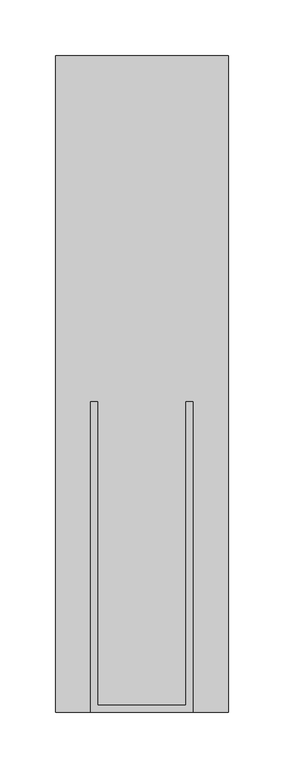
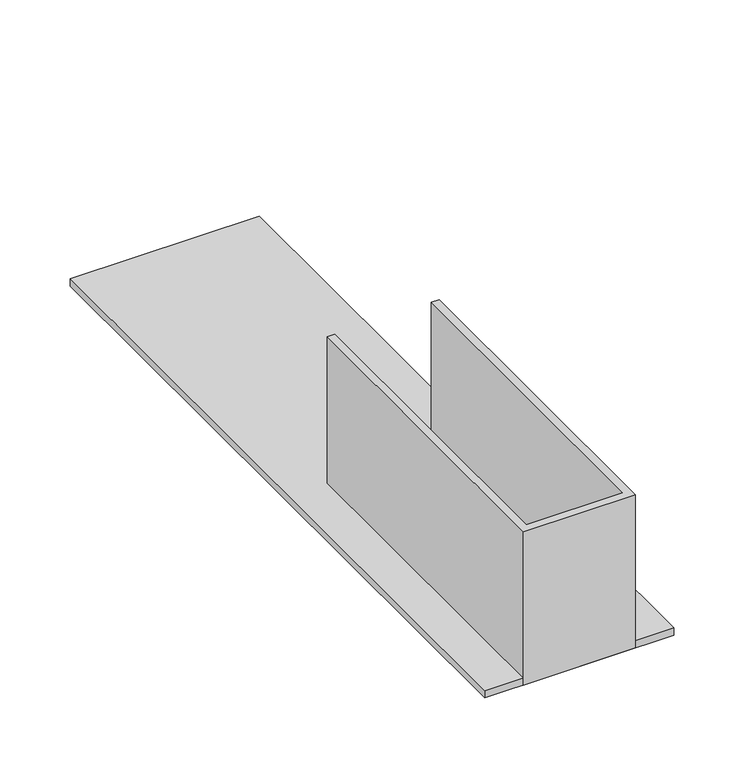
"""IFC4 building model written with IfcOpenShell, lengths in millimetres: fastener geometry, SIMPSON -THGBV - Truss Girder Hanger : SIMPSON -THGBV3.62/11 - HDG."""

import ifcopenshell
import ifcopenshell.guid

model = None  # the IFC model being written
_history = None  # IfcOwnerHistory: only IFC2X3 demands one
_inside = {}  # id of a spatial element -> (the spatial element, [elements in it])
_under = {}  # id of a project, library or spatial element -> (it, [spatial elements below it])
_declared = {}  # id of a project -> (the project, [libraries it declares])
_typed = {}  # id of a type object -> (the type object, [elements of that type])
_made_of = {}  # id of a material, layer set ... -> (it, [elements and type objects made of it])


def new_model(schema):
    """Start an empty IFC model of exactly this schema.

    Asked for "IFC4X3", IfcOpenShell would pick the latest addendum, in which some entities
    have other attributes; the version numbers below select the first issue.
    IFC2X3 requires an IfcOwnerHistory on every rooted entity: one is made here for all.
    """
    global model, _history
    if schema == "IFC4X3":
        model = ifcopenshell.file(schema_version=(4, 3, 0, 0))
    else:
        model = ifcopenshell.file(schema=schema)
    _inside.clear()
    _under.clear()
    _declared.clear()
    _typed.clear()
    _made_of.clear()
    _history = None
    if model.schema == "IFC2X3":
        org = make("IfcOrganization", Name="unknown")
        user = make(
            "IfcPersonAndOrganization",
            ThePerson=make("IfcPerson", FamilyName="unknown"),
            TheOrganization=org,
        )
        app = make(
            "IfcApplication",
            ApplicationDeveloper=org,
            Version="unknown",
            ApplicationFullName="unknown",
            ApplicationIdentifier="unknown",
        )
        _history = make(
            "IfcOwnerHistory",
            OwningUser=user,
            OwningApplication=app,
            ChangeAction="ADDED",
            CreationDate=0,
        )
    return model


def make(cls, **values):
    """One entity of the class cls with the attributes given. An attribute that is None is left unset."""
    return model.create_entity(
        cls, **{name: value for name, value in values.items() if value is not None}
    )


def rooted(cls, **values):
    """An entity with a GlobalId (a new one), such as an element, a storey or a relation."""
    return make(cls, GlobalId=ifcopenshell.guid.new(), OwnerHistory=_history, **values)


def si_unit(unit_type, name, prefix=None):
    """IfcSIUnit, for example si_unit("LENGTHUNIT", "METRE", prefix="MILLI")."""
    return make("IfcSIUnit", UnitType=unit_type, Prefix=prefix, Name=name)


def assignment(units):
    """IfcUnitAssignment: the units of a project."""
    return None if units is None else make("IfcUnitAssignment", Units=units)


def point(xyz):
    """IfcCartesianPoint."""
    return None if xyz is None else make("IfcCartesianPoint", Coordinates=xyz)


def direction(xyz):
    """IfcDirection."""
    return None if xyz is None else make("IfcDirection", DirectionRatios=xyz)


def frame(location, z_axis=None, x_axis=None):
    """IfcAxis2Placement3D, a coordinate frame: its origin and axes. An axis left out is left unset."""
    return make(
        "IfcAxis2Placement3D",
        Location=point(location),
        Axis=direction(z_axis),
        RefDirection=direction(x_axis),
    )


def origin():
    """The frame at (0, 0, 0) with its axes left unset."""
    return frame((0.0, 0.0, 0.0))


def origin_with_axes():
    """The frame at (0, 0, 0) with the z axis (0, 0, 1) and the x axis (1, 0, 0) written out."""
    return frame((0.0, 0.0, 0.0), z_axis=(0.0, 0.0, 1.0), x_axis=(1.0, 0.0, 0.0))


def place(relative_to, where):
    """IfcLocalPlacement: puts the frame where relative to a parent placement (None: the world)."""
    return make(
        "IfcLocalPlacement", PlacementRelTo=relative_to, RelativePlacement=where
    )


def context(
    kind, dimensions, precision=None, world=None, true_north=None, identifier=None
):
    """IfcGeometricRepresentationContext, for example the 3D "Model" context."""
    return make(
        "IfcGeometricRepresentationContext",
        ContextIdentifier=identifier,
        ContextType=kind,
        CoordinateSpaceDimension=dimensions,
        Precision=precision,
        WorldCoordinateSystem=world,
        TrueNorth=true_north,
    )


def project(units=None, contexts=None):
    """IfcProject with its units and contexts."""
    return rooted(
        "IfcProject",
        Name="project",
        RepresentationContexts=contexts,
        UnitsInContext=assignment(units),
    )


def spatial(cls, under=None, at=None, **own):
    """A site, building, storey or space (cls), placed at a placement, below another one or the project."""
    s = rooted(cls, ObjectPlacement=at, **own)
    if under is not None:
        _under.setdefault(under.id(), (under, []))[1].append(s)
    return s


def polyline(points):
    """IfcPolyline through the points."""
    return make("IfcPolyline", Points=[point(p) for p in points])


def outline(outer, holes=None, kind="AREA"):
    """IfcArbitraryClosedProfileDef: a profile drawn as a closed curve; with holes, ...WithVoids."""
    if holes is None:
        return make("IfcArbitraryClosedProfileDef", ProfileType=kind, OuterCurve=outer)
    return make(
        "IfcArbitraryProfileDefWithVoids",
        ProfileType=kind,
        OuterCurve=outer,
        InnerCurves=holes,
    )


def extrude(swept, where, along, depth):
    """IfcExtrudedAreaSolid: the profile swept, set in the frame where, extruded along a direction by depth."""
    return make(
        "IfcExtrudedAreaSolid",
        SweptArea=swept,
        Position=where,
        ExtrudedDirection=direction(along),
        Depth=depth,
    )


def shape(context_of_items, identifier, shape_type, items):
    """IfcShapeRepresentation: the items that make up one representation, for example the "Body"."""
    return make(
        "IfcShapeRepresentation",
        ContextOfItems=context_of_items,
        RepresentationIdentifier=identifier,
        RepresentationType=shape_type,
        Items=items,
    )


def source(mapping_origin, context_of_items, identifier, shape_type, items):
    """IfcRepresentationMap: a shape defined once, which mapped items show again and again."""
    return make(
        "IfcRepresentationMap",
        MappingOrigin=mapping_origin,
        MappedRepresentation=shape(context_of_items, identifier, shape_type, items),
    )


def transform(
    local_origin,
    x_axis=None,
    y_axis=None,
    z_axis=None,
    scale=None,
    scale2=None,
    scale3=None,
    uniform=True,
):
    """IfcCartesianTransformationOperator3D, or its non-uniform kind. x_axis, y_axis, z_axis: its Axis1, 2, 3."""
    if uniform:
        return make(
            "IfcCartesianTransformationOperator3D",
            Axis1=direction(x_axis),
            Axis2=direction(y_axis),
            LocalOrigin=point(local_origin),
            Scale=scale,
            Axis3=direction(z_axis),
        )
    return make(
        "IfcCartesianTransformationOperator3DnonUniform",
        Axis1=direction(x_axis),
        Axis2=direction(y_axis),
        LocalOrigin=point(local_origin),
        Scale=scale,
        Axis3=direction(z_axis),
        Scale2=scale2,
        Scale3=scale3,
    )


def mapped(mapping_source, mapping_target):
    """IfcMappedItem: shows the shape of a source again, moved by a transform."""
    return make(
        "IfcMappedItem", MappingSource=mapping_source, MappingTarget=mapping_target
    )


def made_of(thing, what):
    """Note that an element or type object is made of a material, layer set ...; save() writes the relation."""
    if what is not None:
        _made_of.setdefault(what.id(), (what, []))[1].append(thing)
    return thing


def element(
    cls,
    number,
    at=None,
    inside=None,
    cuts=None,
    type_object=None,
    material=None,
    context=None,
    identifier="Body",
    shape_type=None,
    held_by="IfcProductDefinitionShape",
    body=None,
    shapes=None,
    **own,
):
    """One element of the class cls, such as IfcWall. Its Tag is "e" and its number.

    at: its placement. inside: the storey or other place that contains it. cuts: it is an
    opening in that element (IfcRelVoidsElement). A single representation is given by context,
    identifier, shape_type and body (its items); several are given by shapes. held_by: the class
    of the entity that holds the representations. save() writes the other relations.
    """
    e = rooted(cls, Tag="e%d" % number, ObjectPlacement=at, **own)
    if body is not None:
        shapes = [shape(context, identifier, shape_type, body)]
    if shapes is not None:
        e.Representation = make(held_by, Representations=shapes)
    if inside is not None:
        _inside.setdefault(inside.id(), (inside, []))[1].append(e)
    if cuts is not None:
        rooted(
            "IfcRelVoidsElement", RelatingBuildingElement=cuts, RelatedOpeningElement=e
        )
    if type_object is not None:
        _typed.setdefault(type_object.id(), (type_object, []))[1].append(e)
    return made_of(e, material)


def aggregate(whole, parts):
    """IfcRelAggregates: a whole, such as a stair, and the parts it consists of."""
    return rooted("IfcRelAggregates", RelatingObject=whole, RelatedObjects=parts)


def save(model, path):
    """Write the relations noted so far, then the file.

    IfcRelAggregates (storeys below a building ...), IfcRelContainedInSpatialStructure (elements
    in a storey), IfcRelDefinesByType, IfcRelAssociatesMaterial and IfcRelDeclares: one each for
    every whole, place, type object, material and project.
    """
    for whole, parts in _under.values():
        aggregate(whole, parts)
    for where, things in _inside.values():
        rooted(
            "IfcRelContainedInSpatialStructure",
            RelatedElements=things,
            RelatingStructure=where,
        )
    for kind, things in _typed.values():
        rooted("IfcRelDefinesByType", RelatedObjects=things, RelatingType=kind)
    for what, things in _made_of.values():
        rooted("IfcRelAssociatesMaterial", RelatedObjects=things, RelatingMaterial=what)
    for by, libraries in _declared.values():
        rooted("IfcRelDeclares", RelatingContext=by, RelatedDefinitions=libraries)
    model.write(path)


def fastener_a0b837a1(model_context):
    return source(origin(), model_context, "Body", "SweptSolid", [
        extrude(outline(polyline([(-46.0375, 0.0), (-46.0375, 279.4), (-39.6875, 279.4), (-39.6875, 6.35), (39.6875, 6.35), (39.6875, 279.4), (46.0375, 279.4), (46.0375, 0.0), (-46.0375, 0.0)])), origin_with_axes(), (0.0, 0.0, 1.0), 133.35),
        extrude(outline(polyline([(77.7875, 590.55), (77.7875, 0.0), (-77.7875, 0.0), (-77.7875, 590.55), (77.7875, 590.55)])), origin_with_axes(), (0.0, 0.0, 1.0), 6.35),
    ])


if __name__ == "__main__":
    model = new_model("IFC4")
    model_context = context("Model", 3, world=origin())
    ifc_project = project(units=[si_unit("LENGTHUNIT", "METRE", prefix="MILLI")], contexts=[model_context])
    site = spatial("IfcSite", under=ifc_project)
    building = spatial("IfcBuilding", under=site)
    placement = place(None, origin())
    fastener_shape = fastener_a0b837a1(model_context)
    element("IfcFastener", 1, ObjectType="SIMPSON -THGBV - Truss Girder Hanger : SIMPSON -THGBV3.62/11 - HDG", at=placement, inside=building, context=model_context, shape_type="MappedRepresentation", body=[
        mapped(fastener_shape, transform((0.0, 0.0, 0.0), x_axis=(1.0, 0.0, 0.0), y_axis=(0.0, 1.0, 0.0), z_axis=(0.0, 0.0, 1.0))),
    ])
    save(model, "model.ifc")

# Revit data of these elements
# Type "SIMPSON -THGBV - Truss Girder Hanger : SIMPSON -THGBV3.62/11 - HDG"
#   URL = "http://embed.widencdn.net/pdf/plus/ssttoolbox/iecrxc4cbv/C-C-2017-p254-255.pdf"
#   W = 0' - 3 5/8"
#   H = 0' - 11"
#   Default Elevation = 4' - 0"
